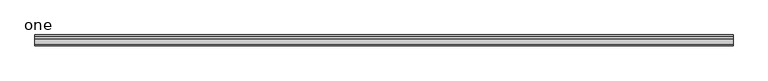
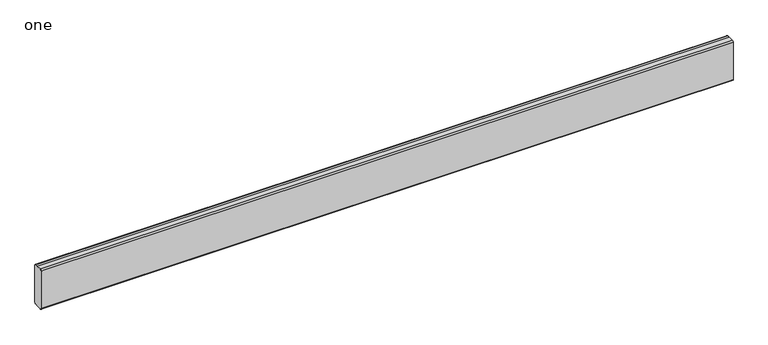
"""IFC4 building model written with IfcOpenShell, lengths in millimetres: beam geometry, Trex : one."""

from ifc_helpers import new_model, si_unit, point, frame, frame_2d, origin, place, context, project, spatial, polyline, circle_curve, trimmed, segment, composite_curve, outline, extrude, source, transform, mapped, element, save


def one_48b49778(model_context):
    return source(origin(), model_context, "Body", "SweptSolid", [
        extrude(outline(composite_curve([segment(polyline([(4.9179935, -103.2371094), (-19.7941406, -103.2371094)]), True, "CONTINUOUS"), segment(trimmed(circle_curve(frame_2d((-19.7941406, -96.8871094)), 6.35), [point((-19.7941406, -103.2371094))], [point((-26.1441406, -96.8871094))], False, "CARTESIAN"), True, "CONTINUOUS"), segment(polyline([(-26.1441406, -96.8871094), (-26.1441406, 96.8871094)]), True, "CONTINUOUS"), segment(trimmed(circle_curve(frame_2d((-19.7941406, 96.8871094)), 6.35), [point((-26.1441406, 96.8871094))], [point((-19.7941406, 103.2371094))], False, "CARTESIAN"), True, "CONTINUOUS"), segment(polyline([(-19.7941406, 103.2371094), (4.9179935, 103.2371094), (4.9179935, 101.6496094), (19.7941406, 101.6496094)]), True, "CONTINUOUS"), segment(trimmed(circle_curve(frame_2d((19.7941406, 95.2996094)), 6.35), [point((19.7941406, 101.6496094))], [point((26.1441406, 95.2996094))], False, "CARTESIAN"), True, "CONTINUOUS"), segment(polyline([(26.1441406, 95.2996094), (26.1441406, -95.2996094)]), True, "CONTINUOUS"), segment(trimmed(circle_curve(frame_2d((19.7941406, -95.2996094)), 6.35), [point((26.1441406, -95.2996094))], [point((19.7941406, -101.6496094))], False, "CARTESIAN"), True, "CONTINUOUS"), segment(polyline([(19.7941406, -101.6496094), (4.9179935, -101.6496094), (4.9179935, -103.2371094)]), True, "CONTINUOUS")], self_intersect=False)), frame((-1692.0711791, 0.0, 0.0), z_axis=(1.0, 0.0, 0.0), x_axis=(0.0, 1.0, 0.0)), (0.0, 0.0, 1.0), 3384.1423581),
    ])


if __name__ == "__main__":
    model = new_model("IFC4")
    model_context = context("Model", 3, world=origin())
    ifc_project = project(units=[si_unit("LENGTHUNIT", "METRE", prefix="MILLI")], contexts=[model_context])
    site = spatial("IfcSite", under=ifc_project)
    building = spatial("IfcBuilding", under=site)
    placement = place(None, origin())
    one_shape = one_48b49778(model_context)
    element("IfcBeam", 1, ObjectType="Trex : one", at=placement, inside=building, context=model_context, shape_type="MappedRepresentation", body=[
        mapped(one_shape, transform((0.0, 0.0, 0.0), x_axis=(1.0, 0.0, 0.0), y_axis=(0.0, 1.0, 0.0), z_axis=(0.0, 0.0, 1.0))),
    ])
    save(model, "model.ifc")

# Revit data of these elements
# Type "Trex : one"
#   Width = 0' - 2 15/256"
#   Web_Thickness = 0' - 0 7/64"
#   Length [instance default] = 10' - 0"
#   Leg_1 = 0' - 2 1/2"
#   Height = 0' - 8 33/256"
#   Structural Material [instance default] = none
